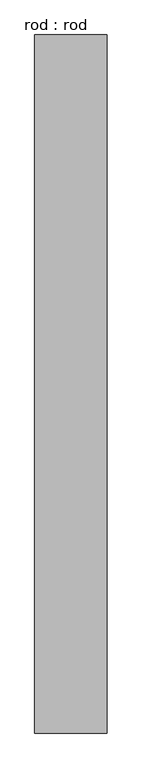
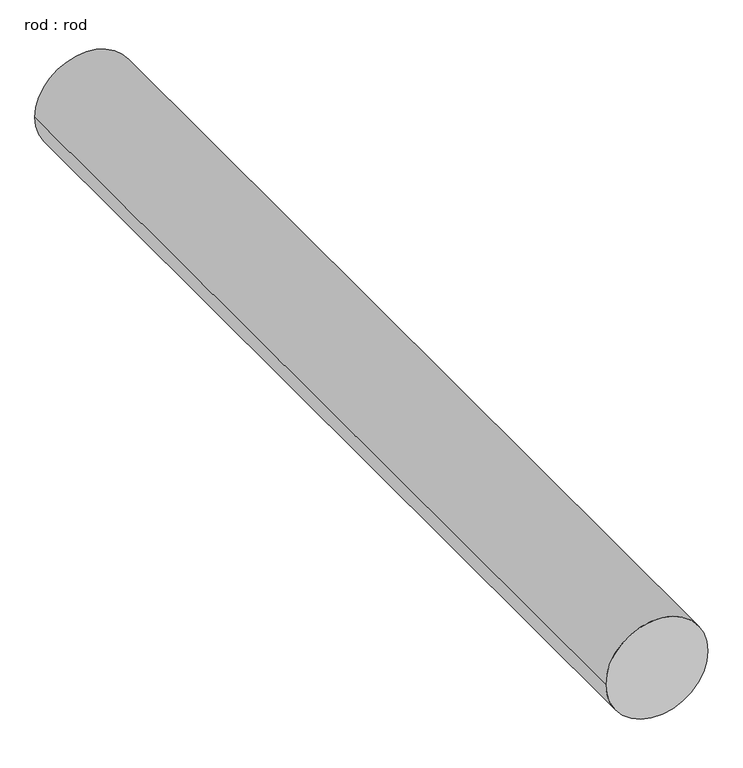
"""IFC4 building model written with IfcOpenShell, lengths in millimetres: proxy geometry, rod : rod."""

import ifcopenshell
import ifcopenshell.guid

model = None  # the IFC model being written
_history = None  # IfcOwnerHistory: only IFC2X3 demands one
_inside = {}  # id of a spatial element -> (the spatial element, [elements in it])
_under = {}  # id of a project, library or spatial element -> (it, [spatial elements below it])
_declared = {}  # id of a project -> (the project, [libraries it declares])
_typed = {}  # id of a type object -> (the type object, [elements of that type])
_made_of = {}  # id of a material, layer set ... -> (it, [elements and type objects made of it])


def new_model(schema):
    """Start an empty IFC model of exactly this schema.

    Asked for "IFC4X3", IfcOpenShell would pick the latest addendum, in which some entities
    have other attributes; the version numbers below select the first issue.
    IFC2X3 requires an IfcOwnerHistory on every rooted entity: one is made here for all.
    """
    global model, _history
    if schema == "IFC4X3":
        model = ifcopenshell.file(schema_version=(4, 3, 0, 0))
    else:
        model = ifcopenshell.file(schema=schema)
    _inside.clear()
    _under.clear()
    _declared.clear()
    _typed.clear()
    _made_of.clear()
    _history = None
    if model.schema == "IFC2X3":
        org = make("IfcOrganization", Name="unknown")
        user = make(
            "IfcPersonAndOrganization",
            ThePerson=make("IfcPerson", FamilyName="unknown"),
            TheOrganization=org,
        )
        app = make(
            "IfcApplication",
            ApplicationDeveloper=org,
            Version="unknown",
            ApplicationFullName="unknown",
            ApplicationIdentifier="unknown",
        )
        _history = make(
            "IfcOwnerHistory",
            OwningUser=user,
            OwningApplication=app,
            ChangeAction="ADDED",
            CreationDate=0,
        )
    return model


def make(cls, **values):
    """One entity of the class cls with the attributes given. An attribute that is None is left unset."""
    return model.create_entity(
        cls, **{name: value for name, value in values.items() if value is not None}
    )


def rooted(cls, **values):
    """An entity with a GlobalId (a new one), such as an element, a storey or a relation."""
    return make(cls, GlobalId=ifcopenshell.guid.new(), OwnerHistory=_history, **values)


def si_unit(unit_type, name, prefix=None):
    """IfcSIUnit, for example si_unit("LENGTHUNIT", "METRE", prefix="MILLI")."""
    return make("IfcSIUnit", UnitType=unit_type, Prefix=prefix, Name=name)


def assignment(units):
    """IfcUnitAssignment: the units of a project."""
    return None if units is None else make("IfcUnitAssignment", Units=units)


def point(xyz):
    """IfcCartesianPoint."""
    return None if xyz is None else make("IfcCartesianPoint", Coordinates=xyz)


def direction(xyz):
    """IfcDirection."""
    return None if xyz is None else make("IfcDirection", DirectionRatios=xyz)


def frame(location, z_axis=None, x_axis=None):
    """IfcAxis2Placement3D, a coordinate frame: its origin and axes. An axis left out is left unset."""
    return make(
        "IfcAxis2Placement3D",
        Location=point(location),
        Axis=direction(z_axis),
        RefDirection=direction(x_axis),
    )


def frame_2d(location, x_axis=None):
    """IfcAxis2Placement2D, a coordinate frame in the plane: its origin and x axis."""
    return make(
        "IfcAxis2Placement2D", Location=point(location), RefDirection=direction(x_axis)
    )


def origin():
    """The frame at (0, 0, 0) with its axes left unset."""
    return frame((0.0, 0.0, 0.0))


def place(relative_to, where):
    """IfcLocalPlacement: puts the frame where relative to a parent placement (None: the world)."""
    return make(
        "IfcLocalPlacement", PlacementRelTo=relative_to, RelativePlacement=where
    )


def context(
    kind, dimensions, precision=None, world=None, true_north=None, identifier=None
):
    """IfcGeometricRepresentationContext, for example the 3D "Model" context."""
    return make(
        "IfcGeometricRepresentationContext",
        ContextIdentifier=identifier,
        ContextType=kind,
        CoordinateSpaceDimension=dimensions,
        Precision=precision,
        WorldCoordinateSystem=world,
        TrueNorth=true_north,
    )


def project(units=None, contexts=None):
    """IfcProject with its units and contexts."""
    return rooted(
        "IfcProject",
        Name="project",
        RepresentationContexts=contexts,
        UnitsInContext=assignment(units),
    )


def spatial(cls, under=None, at=None, **own):
    """A site, building, storey or space (cls), placed at a placement, below another one or the project."""
    s = rooted(cls, ObjectPlacement=at, **own)
    if under is not None:
        _under.setdefault(under.id(), (under, []))[1].append(s)
    return s


def circle_curve(where, radius):
    """IfcCircle in the frame where."""
    return make("IfcCircle", Position=where, Radius=radius)


def trimmed(basis, trim1, trim2, sense, master):
    """IfcTrimmedCurve: the piece of a basis curve between two trims."""
    return make(
        "IfcTrimmedCurve",
        BasisCurve=basis,
        Trim1=trim1,
        Trim2=trim2,
        SenseAgreement=sense,
        MasterRepresentation=master,
    )


def segment(curve, same_sense, transition):
    """IfcCompositeCurveSegment."""
    return make(
        "IfcCompositeCurveSegment",
        Transition=transition,
        SameSense=same_sense,
        ParentCurve=curve,
    )


def composite_curve(segments, self_intersect=None):
    """IfcCompositeCurve: segments joined end to end."""
    return make("IfcCompositeCurve", Segments=segments, SelfIntersect=self_intersect)


def outline(outer, holes=None, kind="AREA"):
    """IfcArbitraryClosedProfileDef: a profile drawn as a closed curve; with holes, ...WithVoids."""
    if holes is None:
        return make("IfcArbitraryClosedProfileDef", ProfileType=kind, OuterCurve=outer)
    return make(
        "IfcArbitraryProfileDefWithVoids",
        ProfileType=kind,
        OuterCurve=outer,
        InnerCurves=holes,
    )


def extrude(swept, where, along, depth):
    """IfcExtrudedAreaSolid: the profile swept, set in the frame where, extruded along a direction by depth."""
    return make(
        "IfcExtrudedAreaSolid",
        SweptArea=swept,
        Position=where,
        ExtrudedDirection=direction(along),
        Depth=depth,
    )


def shape(context_of_items, identifier, shape_type, items):
    """IfcShapeRepresentation: the items that make up one representation, for example the "Body"."""
    return make(
        "IfcShapeRepresentation",
        ContextOfItems=context_of_items,
        RepresentationIdentifier=identifier,
        RepresentationType=shape_type,
        Items=items,
    )


def source(mapping_origin, context_of_items, identifier, shape_type, items):
    """IfcRepresentationMap: a shape defined once, which mapped items show again and again."""
    return make(
        "IfcRepresentationMap",
        MappingOrigin=mapping_origin,
        MappedRepresentation=shape(context_of_items, identifier, shape_type, items),
    )


def transform(
    local_origin,
    x_axis=None,
    y_axis=None,
    z_axis=None,
    scale=None,
    scale2=None,
    scale3=None,
    uniform=True,
):
    """IfcCartesianTransformationOperator3D, or its non-uniform kind. x_axis, y_axis, z_axis: its Axis1, 2, 3."""
    if uniform:
        return make(
            "IfcCartesianTransformationOperator3D",
            Axis1=direction(x_axis),
            Axis2=direction(y_axis),
            LocalOrigin=point(local_origin),
            Scale=scale,
            Axis3=direction(z_axis),
        )
    return make(
        "IfcCartesianTransformationOperator3DnonUniform",
        Axis1=direction(x_axis),
        Axis2=direction(y_axis),
        LocalOrigin=point(local_origin),
        Scale=scale,
        Axis3=direction(z_axis),
        Scale2=scale2,
        Scale3=scale3,
    )


def mapped(mapping_source, mapping_target):
    """IfcMappedItem: shows the shape of a source again, moved by a transform."""
    return make(
        "IfcMappedItem", MappingSource=mapping_source, MappingTarget=mapping_target
    )


def made_of(thing, what):
    """Note that an element or type object is made of a material, layer set ...; save() writes the relation."""
    if what is not None:
        _made_of.setdefault(what.id(), (what, []))[1].append(thing)
    return thing


def element(
    cls,
    number,
    at=None,
    inside=None,
    cuts=None,
    type_object=None,
    material=None,
    context=None,
    identifier="Body",
    shape_type=None,
    held_by="IfcProductDefinitionShape",
    body=None,
    shapes=None,
    **own,
):
    """One element of the class cls, such as IfcWall. Its Tag is "e" and its number.

    at: its placement. inside: the storey or other place that contains it. cuts: it is an
    opening in that element (IfcRelVoidsElement). A single representation is given by context,
    identifier, shape_type and body (its items); several are given by shapes. held_by: the class
    of the entity that holds the representations. save() writes the other relations.
    """
    e = rooted(cls, Tag="e%d" % number, ObjectPlacement=at, **own)
    if body is not None:
        shapes = [shape(context, identifier, shape_type, body)]
    if shapes is not None:
        e.Representation = make(held_by, Representations=shapes)
    if inside is not None:
        _inside.setdefault(inside.id(), (inside, []))[1].append(e)
    if cuts is not None:
        rooted(
            "IfcRelVoidsElement", RelatingBuildingElement=cuts, RelatedOpeningElement=e
        )
    if type_object is not None:
        _typed.setdefault(type_object.id(), (type_object, []))[1].append(e)
    return made_of(e, material)


def aggregate(whole, parts):
    """IfcRelAggregates: a whole, such as a stair, and the parts it consists of."""
    return rooted("IfcRelAggregates", RelatingObject=whole, RelatedObjects=parts)


def save(model, path):
    """Write the relations noted so far, then the file.

    IfcRelAggregates (storeys below a building ...), IfcRelContainedInSpatialStructure (elements
    in a storey), IfcRelDefinesByType, IfcRelAssociatesMaterial and IfcRelDeclares: one each for
    every whole, place, type object, material and project.
    """
    for whole, parts in _under.values():
        aggregate(whole, parts)
    for where, things in _inside.values():
        rooted(
            "IfcRelContainedInSpatialStructure",
            RelatedElements=things,
            RelatingStructure=where,
        )
    for kind, things in _typed.values():
        rooted("IfcRelDefinesByType", RelatedObjects=things, RelatingType=kind)
    for what, things in _made_of.values():
        rooted("IfcRelAssociatesMaterial", RelatedObjects=things, RelatingMaterial=what)
    for by, libraries in _declared.values():
        rooted("IfcRelDeclares", RelatingContext=by, RelatedDefinitions=libraries)
    model.write(path)


def rod_rod_64291a28(model_context):
    return source(origin(), model_context, "Body", "SweptSolid", [
        extrude(outline(composite_curve([segment(trimmed(circle_curve(frame_2d((0.0108462, 0.0)), 200.0), [point((0.0108462, 200.0))], [point((0.0108462, -200.0))], False, "CARTESIAN"), True, "CONTINUOUS"), segment(trimmed(circle_curve(frame_2d((0.0108462, 0.0)), 200.0), [point((0.0108462, -200.0))], [point((0.0108462, 200.0))], False, "CARTESIAN"), True, "CONTINUOUS")], self_intersect=False)), frame((0.0, 2160.7461491, 0.0), z_axis=(0.0, 1.0, 0.0), x_axis=(0.0, 0.0, 1.0)), (0.0, 0.0, 1.0), 3863.9649326),
    ])


if __name__ == "__main__":
    model = new_model("IFC4")
    model_context = context("Model", 3, world=origin())
    ifc_project = project(units=[si_unit("LENGTHUNIT", "METRE", prefix="MILLI")], contexts=[model_context])
    site = spatial("IfcSite", under=ifc_project)
    building = spatial("IfcBuilding", under=site)
    placement = place(None, origin())
    rod_rod_shape = rod_rod_64291a28(model_context)
    element("IfcBuildingElementProxy", 1, Name="rod : rod", ObjectType="rod : rod", at=placement, inside=building, context=model_context, shape_type="MappedRepresentation", body=[
        mapped(rod_rod_shape, transform((0.0, 0.0, 0.0), x_axis=(1.0, 0.0, 0.0), y_axis=(0.0, 1.0, 0.0), z_axis=(0.0, 0.0, 1.0))),
    ])
    save(model, "model.ifc")

# Revit data of these elements
# Type "rod : rod"
#   Default Elevation = 0
